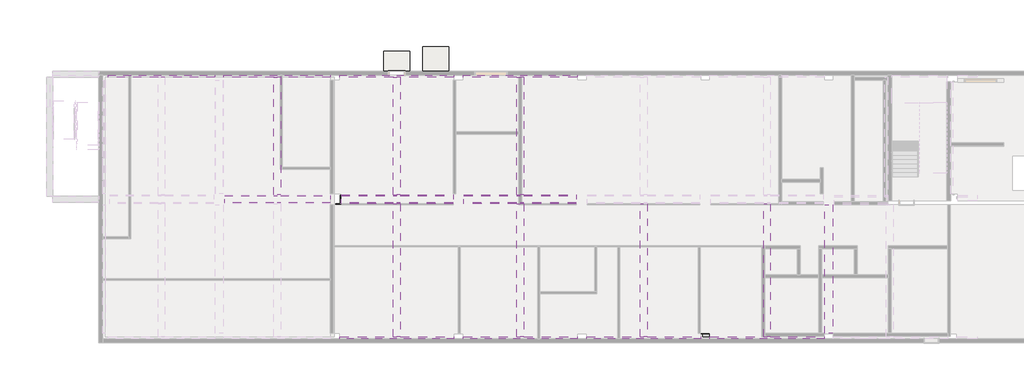
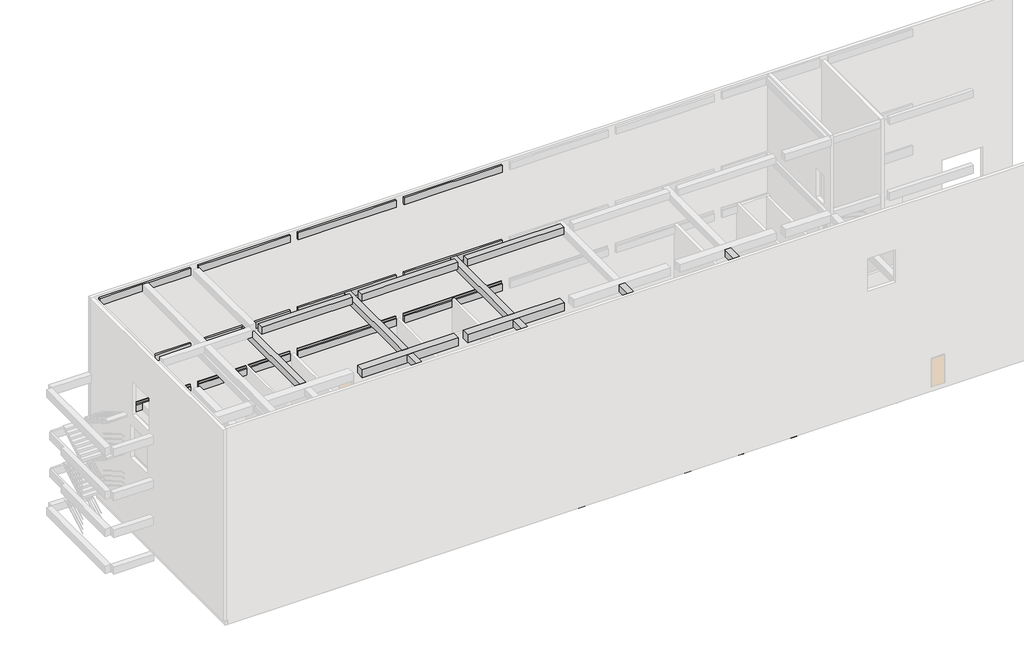
# One storey, part 3 of 5: 54 beams, 2 slabs.
# Revit data of these elements (continued)
# Type "RC Beam_Rectangular : H_SB_AR_S16_UG_B600xH800_1G2" (continued)
#   H_WM Code_1 = "A03AF032-00022 |  | M3 | Concrete Work | Superstructure Work | Structural Concrete | Cement Type-1 | 25MPa ≤ F'c (Cylinder Strength) < 30MPa |  |  |  |  | A03AF032-00022 Concrete Work Superstructure Work Structural Concrete  Cement Type-1 25MPa ≤ F'c (Cylinder Strength) < 30MPa      |  F'c (Cylinder Strength) = 24MPa"
#   H_WM Code_2 = "A03AD037-00002 |  | TON | Concrete Work | Substructure Work | Rebar Work | Deformed Bar (Non-Coat.) | 400MPa<Fy≤470MPa |  |  |  |  | A03AD037-00002 Concrete Work Substructure Work Rebar Work Deformed Bar (Non-Coat.)  400MPa<Fy≤470MPa      | ASTM A615 GRADE 60 (Fy=420MPa)"
#   H_WM Code_3 = "A03AF036-00001 |  | M2 | Concrete Work | Superstructure Work | Form Work (1 time in use) | Flat Form | Dressed Lumber, Plywood or Steel Form(Wood Planks are not Allowed) incl. Chamfer |  |  |  | A03AF036-00001 Concrete Work Superstructure Work Form Work (1 time in use) Flat Form     Dressed Lumber, Plywood or Steel Form(Wood Planks are not Allowed) incl. Chamfer   |"
#   중앙부 하부근 = ""
#   중앙부 상부근 = ""
#   중앙부 보조근 = ""
#   중앙부 늑근 = ""
#   외단부 하부근 = ""
#   외단부 상부근 = ""
#   외단부 보조근 = ""
#   외단부 늑근 = ""
#   부호 = "TG2"
#   내단부 하부근 = ""
#   내단부 상부근 = ""
#   내단부 보조근 = ""
#   내단부 늑근 = ""
#   ALL 하부근 = "3-D20"
#   ALL 상부근 = "4-D20"
#   ALL 보조근 = ""
#   ALL 늑근 = "2-D10 @120"
#   H_Rebar ratio = 0.14
#   Width = 600 mm
#   Height = 800 mm
#   Length [instance default] = 1524 mm
#   b = 600 mm
#   h = 800 mm
#   hec_material3 [instance default] = none
#   hec_material2 [instance default] = none
#   hec_material1 [instance default] = none
#   Structural Material [instance default] = none
#   Assembly Code = ""
# Type "RC Beam_Rectangular : H_SB_AR_S16_UG_B450xH700_1B1"
#   Type Comments = "CV-UG"
#   Type Mark = "1B1"
#   H_Q'ty Cal Type Tag = "SB-Q1"
#   H_WM Code_1 = "A03AF032-00022 |  | M3 | Concrete Work | Superstructure Work | Structural Concrete | Cement Type-1 | 25MPa ≤ F'c (Cylinder Strength) < 30MPa |  |  |  |  | A03AF032-00022 Concrete Work Superstructure Work Structural Concrete  Cement Type-1 25MPa ≤ F'c (Cylinder Strength) < 30MPa      |  F'c (Cylinder Strength) = 24MPa"
#   H_WM Code_2 = "A03AD037-00002 |  | TON | Concrete Work | Substructure Work | Rebar Work | Deformed Bar (Non-Coat.) | 400MPa<Fy≤470MPa |  |  |  |  | A03AD037-00002 Concrete Work Substructure Work Rebar Work Deformed Bar (Non-Coat.)  400MPa<Fy≤470MPa      | ASTM A615 GRADE 60 (Fy=420MPa)"
#   H_WM Code_3 = "A03AF036-00001 |  | M2 | Concrete Work | Superstructure Work | Form Work (1 time in use) | Flat Form | Dressed Lumber, Plywood or Steel Form(Wood Planks are not Allowed) incl. Chamfer |  |  |  | A03AF036-00001 Concrete Work Superstructure Work Form Work (1 time in use) Flat Form     Dressed Lumber, Plywood or Steel Form(Wood Planks are not Allowed) incl. Chamfer   |"
#   중앙부 하부근 = ""
#   중앙부 상부근 = ""
#   중앙부 보조근 = ""
#   중앙부 늑근 = ""
#   외단부 하부근 = ""
#   외단부 상부근 = ""
#   외단부 보조근 = ""
#   외단부 늑근 = ""
#   부호 = "TG2"
#   내단부 하부근 = ""
#   내단부 상부근 = ""
#   내단부 보조근 = ""
#   내단부 늑근 = ""
#   ALL 하부근 = "3-D20"
#   ALL 상부근 = "4-D20"
#   ALL 보조근 = ""
#   ALL 늑근 = "2-D10 @120"
#   H_Rebar ratio = 0.14
#   Width = 450 mm
#   Height = 700 mm
#   Length [instance default] = 1524 mm
#   b = 450 mm
#   h = 700 mm
#   hec_material3 [instance default] = none
#   hec_material2 [instance default] = none
#   hec_material1 [instance default] = none
#   Structural Material [instance default] = none
#   Assembly Code = ""
# Type "RC Beam_Rectangular : H_SB_AR_S16_UG_B500xH700_1G1"
#   Type Comments = "CV-UG"
#   Type Mark = "1G1"
#   H_Q'ty Cal Type Tag = "SB-Q1"
#   H_WM Code_1 = "A03AF032-00022 |  | M3 | Concrete Work | Superstructure Work | Structural Concrete | Cement Type-1 | 25MPa ≤ F'c (Cylinder Strength) < 30MPa |  |  |  |  | A03AF032-00022 Concrete Work Superstructure Work Structural Concrete  Cement Type-1 25MPa ≤ F'c (Cylinder Strength) < 30MPa      |  F'c (Cylinder Strength) = 24MPa"
#   H_WM Code_2 = "A03AD037-00002 |  | TON | Concrete Work | Substructure Work | Rebar Work | Deformed Bar (Non-Coat.) | 400MPa<Fy≤470MPa |  |  |  |  | A03AD037-00002 Concrete Work Substructure Work Rebar Work Deformed Bar (Non-Coat.)  400MPa<Fy≤470MPa      | ASTM A615 GRADE 60 (Fy=420MPa)"
#   H_WM Code_3 = "A03AF036-00001 |  | M2 | Concrete Work | Superstructure Work | Form Work (1 time in use) | Flat Form | Dressed Lumber, Plywood or Steel Form(Wood Planks are not Allowed) incl. Chamfer |  |  |  | A03AF036-00001 Concrete Work Superstructure Work Form Work (1 time in use) Flat Form     Dressed Lumber, Plywood or Steel Form(Wood Planks are not Allowed) incl. Chamfer   |"
#   중앙부 하부근 = ""
#   중앙부 상부근 = ""
#   중앙부 보조근 = ""
#   중앙부 늑근 = ""
#   외단부 하부근 = ""
#   외단부 상부근 = ""
#   외단부 보조근 = ""
#   외단부 늑근 = ""
#   부호 = "TG2"
#   내단부 하부근 = ""
#   내단부 상부근 = ""
#   내단부 보조근 = ""
#   내단부 늑근 = ""
#   ALL 하부근 = "3-D20"
#   ALL 상부근 = "4-D20"
#   ALL 보조근 = ""
#   ALL 늑근 = "2-D10 @120"
#   H_Rebar ratio = 0.14
#   Width = 500 mm
#   Height = 700 mm
#   Length [instance default] = 1524 mm
#   b = 500 mm
#   h = 700 mm
#   hec_material3 [instance default] = none
#   hec_material2 [instance default] = none
#   hec_material1 [instance default] = none
#   Structural Material [instance default] = none
#   Assembly Code = ""
# Type "RC Beam_Rectangular : H_SB_AR_S16_UG_B450xH700_1B1A"
#   Type Comments = "UG"
#   Type Mark = "1B1A"
#   H_Q'ty Cal Type Tag = "SB-Q1"
#   H_WM Code_1 = "A03AF032-00022 |  | M3 | Concrete Work | Superstructure Work | Structural Concrete | Cement Type-1 | 25MPa ≤ F'c (Cylinder Strength) < 30MPa |  |  |  |  | A03AF032-00022 Concrete Work Superstructure Work Structural Concrete  Cement Type-1 25MPa ≤ F'c (Cylinder Strength) < 30MPa      |  F'c (Cylinder Strength) = 24MPa"
#   H_WM Code_2 = "A03AD037-00002 |  | TON | Concrete Work | Substructure Work | Rebar Work | Deformed Bar (Non-Coat.) | 400MPa<Fy≤470MPa |  |  |  |  | A03AD037-00002 Concrete Work Substructure Work Rebar Work Deformed Bar (Non-Coat.)  400MPa<Fy≤470MPa      | ASTM A615 GRADE 60 (Fy=420MPa)"
#   H_WM Code_3 = "A03AF036-00001 |  | M2 | Concrete Work | Superstructure Work | Form Work (1 time in use) | Flat Form | Dressed Lumber, Plywood or Steel Form(Wood Planks are not Allowed) incl. Chamfer |  |  |  | A03AF036-00001 Concrete Work Superstructure Work Form Work (1 time in use) Flat Form     Dressed Lumber, Plywood or Steel Form(Wood Planks are not Allowed) incl. Chamfer   |"
#   중앙부 하부근 = ""
#   중앙부 상부근 = ""
#   중앙부 보조근 = ""
#   중앙부 늑근 = ""
#   외단부 하부근 = ""
#   외단부 상부근 = ""
#   외단부 보조근 = ""
#   외단부 늑근 = ""
#   부호 = "TG2"
#   내단부 하부근 = ""
#   내단부 상부근 = ""
#   내단부 보조근 = ""
#   내단부 늑근 = ""
#   ALL 하부근 = "3-D20"
#   ALL 상부근 = "4-D20"
#   ALL 보조근 = ""
#   ALL 늑근 = "2-D10 @120"
#   Width = 450 mm
#   Height = 700 mm
#   Length [instance default] = 1524 mm
#   b = 450 mm
#   h = 700 mm
#   hec_material3 [instance default] = none
#   hec_material2 [instance default] = none
#   hec_material1 [instance default] = none
#   Structural Material [instance default] = none
#   Assembly Code = ""
# Type "RC Beam_Rectangular : H_SB_AR_S16_AG_B400xH700_3WG1"
#   Type Comments = "CV-AG"
#   Type Mark = "3WG1"
#   H_Q'ty Cal Type Tag = "SB-Q1"
#   H_WM Code_1 = "A03AF032-00022 |  | M3 | Concrete Work | Superstructure Work | Structural Concrete | Cement Type-1 | 25MPa ≤ F'c (Cylinder Strength) < 30MPa |  |  |  |  | A03AF032-00022 Concrete Work Superstructure Work Structural Concrete  Cement Type-1 25MPa ≤ F'c (Cylinder Strength) < 30MPa      |  F'c (Cylinder Strength) = 24MPa"
#   H_WM Code_2 = "A03AD037-00002 |  | TON | Concrete Work | Substructure Work | Rebar Work | Deformed Bar (Non-Coat.) | 400MPa<Fy≤470MPa |  |  |  |  | A03AD037-00002 Concrete Work Substructure Work Rebar Work Deformed Bar (Non-Coat.)  400MPa<Fy≤470MPa      | ASTM A615 GRADE 60 (Fy=420MPa)"
#   H_WM Code_3 = "A03AF036-00001 |  | M2 | Concrete Work | Superstructure Work | Form Work (1 time in use) | Flat Form | Dressed Lumber, Plywood or Steel Form(Wood Planks are not Allowed) incl. Chamfer |  |  |  | A03AF036-00001 Concrete Work Superstructure Work Form Work (1 time in use) Flat Form     Dressed Lumber, Plywood or Steel Form(Wood Planks are not Allowed) incl. Chamfer   |"
#   중앙부 하부근 = ""
#   중앙부 상부근 = ""
#   중앙부 보조근 = ""
#   중앙부 늑근 = ""
#   외단부 하부근 = ""
#   외단부 상부근 = ""
#   외단부 보조근 = ""
#   외단부 늑근 = ""
#   부호 = "TG2"
#   내단부 하부근 = ""
#   내단부 상부근 = ""
#   내단부 보조근 = ""
#   내단부 늑근 = ""
#   ALL 하부근 = "3-D20"
#   ALL 상부근 = "4-D20"
#   ALL 보조근 = ""
#   ALL 늑근 = "2-D10 @120"
#   H_Rebar ratio = 0.14
#   Width = 400 mm
#   Height = 700 mm
#   Length [instance default] = 1524 mm
#   b = 400 mm
#   h = 700 mm
#   hec_material3 [instance default] = none
#   hec_material2 [instance default] = none
#   hec_material1 [instance default] = none
#   Structural Material [instance default] = none
#   Assembly Code = ""
# Type "RC Beam_Rectangular : H_SB_AR_S16_AG_B600xH800_3G2"
#   Type Comments = "AG"
#   Type Mark = "3G2"
#   H_Q'ty Cal Type Tag = "SB-Q1"
#   H_WM Code_1 = "A03AF032-00022 |  | M3 | Concrete Work | Superstructure Work | Structural Concrete | Cement Type-1 | 25MPa ≤ F'c (Cylinder Strength) < 30MPa |  |  |  |  | A03AF032-00022 Concrete Work Superstructure Work Structural Concrete  Cement Type-1 25MPa ≤ F'c (Cylinder Strength) < 30MPa      |  F'c (Cylinder Strength) = 24MPa"
#   H_WM Code_2 = "A03AD037-00002 |  | TON | Concrete Work | Substructure Work | Rebar Work | Deformed Bar (Non-Coat.) | 400MPa<Fy≤470MPa |  |  |  |  | A03AD037-00002 Concrete Work Substructure Work Rebar Work Deformed Bar (Non-Coat.)  400MPa<Fy≤470MPa      | ASTM A615 GRADE 60 (Fy=420MPa)"
#   H_WM Code_3 = "A03AF036-00001 |  | M2 | Concrete Work | Superstructure Work | Form Work (1 time in use) | Flat Form | Dressed Lumber, Plywood or Steel Form(Wood Planks are not Allowed) incl. Chamfer |  |  |  | A03AF036-00001 Concrete Work Superstructure Work Form Work (1 time in use) Flat Form     Dressed Lumber, Plywood or Steel Form(Wood Planks are not Allowed) incl. Chamfer   |"
#   중앙부 하부근 = ""
#   중앙부 상부근 = ""
#   중앙부 보조근 = ""
#   중앙부 늑근 = ""
#   외단부 하부근 = ""
#   외단부 상부근 = ""
#   외단부 보조근 = ""
#   외단부 늑근 = ""
#   부호 = "TG2"
#   내단부 하부근 = ""
#   내단부 상부근 = ""
#   내단부 보조근 = ""
#   내단부 늑근 = ""
#   ALL 하부근 = "3-D20"
#   ALL 상부근 = "4-D20"
#   ALL 보조근 = ""
#   ALL 늑근 = "2-D10 @120"
#   Width = 600 mm
#   Height = 800 mm
#   Length [instance default] = 1524 mm
#   b = 600 mm
#   h = 800 mm
#   hec_material3 [instance default] = none
#   hec_material2 [instance default] = none
#   hec_material1 [instance default] = none
#   Structural Material [instance default] = none
#   Assembly Code = ""
# Type "RC Beam_Rectangular : H_SB_AR_S16_AG_B4500xH700_3G1"
#   Type Comments = "AG"
#   Type Mark = "3G1"
#   H_Q'ty Cal Type Tag = "SB-Q1"
#   H_WM Code_1 = "A03AF032-00022 |  | M3 | Concrete Work | Superstructure Work | Structural Concrete | Cement Type-1 | 25MPa ≤ F'c (Cylinder Strength) < 30MPa |  |  |  |  | A03AF032-00022 Concrete Work Superstructure Work Structural Concrete  Cement Type-1 25MPa ≤ F'c (Cylinder Strength) < 30MPa      |  F'c (Cylinder Strength) = 24MPa"
#   H_WM Code_2 = "A03AD037-00002 |  | TON | Concrete Work | Substructure Work | Rebar Work | Deformed Bar (Non-Coat.) | 400MPa<Fy≤470MPa |  |  |  |  | A03AD037-00002 Concrete Work Substructure Work Rebar Work Deformed Bar (Non-Coat.)  400MPa<Fy≤470MPa      | ASTM A615 GRADE 60 (Fy=420MPa)"
#   H_WM Code_3 = "A03AF036-00001 |  | M2 | Concrete Work | Superstructure Work | Form Work (1 time in use) | Flat Form | Dressed Lumber, Plywood or Steel Form(Wood Planks are not Allowed) incl. Chamfer |  |  |  | A03AF036-00001 Concrete Work Superstructure Work Form Work (1 time in use) Flat Form     Dressed Lumber, Plywood or Steel Form(Wood Planks are not Allowed) incl. Chamfer   |"
#   중앙부 하부근 = ""
#   중앙부 상부근 = ""
#   중앙부 보조근 = ""
#   중앙부 늑근 = ""
#   외단부 하부근 = ""
#   외단부 상부근 = ""
#   외단부 보조근 = ""
#   외단부 늑근 = ""
#   부호 = "TG2"
#   내단부 하부근 = ""
#   내단부 상부근 = ""
#   내단부 보조근 = ""
#   내단부 늑근 = ""
#   ALL 하부근 = "3-D20"
#   ALL 상부근 = "4-D20"
#   ALL 보조근 = ""
#   ALL 늑근 = "2-D10 @120"
#   Width = 500 mm
#   Height = 700 mm
#   Length [instance default] = 1524 mm
#   b = 500 mm
#   h = 700 mm
#   hec_material3 [instance default] = none
#   hec_material2 [instance default] = none
#   hec_material1 [instance default] = none
#   Structural Material [instance default] = none
#   Assembly Code = ""
# Type "RC Beam_Rectangular : H_SB_AR_S16_AG_B450xH700_3B1"
#   Type Comments = "AG"
#   Type Mark = "3B1"
#   H_Q'ty Cal Type Tag = "SB-Q1"
#   H_WM Code_1 = "A03AF032-00022 |  | M3 | Concrete Work | Superstructure Work | Structural Concrete | Cement Type-1 | 25MPa ≤ F'c (Cylinder Strength) < 30MPa |  |  |  |  | A03AF032-00022 Concrete Work Superstructure Work Structural Concrete  Cement Type-1 25MPa ≤ F'c (Cylinder Strength) < 30MPa      |  F'c (Cylinder Strength) = 24MPa"
#   H_WM Code_2 = "A03AD037-00002 |  | TON | Concrete Work | Substructure Work | Rebar Work | Deformed Bar (Non-Coat.) | 400MPa<Fy≤470MPa |  |  |  |  | A03AD037-00002 Concrete Work Substructure Work Rebar Work Deformed Bar (Non-Coat.)  400MPa<Fy≤470MPa      | ASTM A615 GRADE 60 (Fy=420MPa)"
#   H_WM Code_3 = "A03AF036-00001 |  | M2 | Concrete Work | Superstructure Work | Form Work (1 time in use) | Flat Form | Dressed Lumber, Plywood or Steel Form(Wood Planks are not Allowed) incl. Chamfer |  |  |  | A03AF036-00001 Concrete Work Superstructure Work Form Work (1 time in use) Flat Form     Dressed Lumber, Plywood or Steel Form(Wood Planks are not Allowed) incl. Chamfer   |"
#   중앙부 하부근 = ""
#   중앙부 상부근 = ""
#   중앙부 보조근 = ""
#   중앙부 늑근 = ""
#   외단부 하부근 = ""
#   외단부 상부근 = ""
#   외단부 보조근 = ""
#   외단부 늑근 = ""
#   부호 = "TG2"
#   내단부 하부근 = ""
#   내단부 상부근 = ""
#   내단부 보조근 = ""
#   내단부 늑근 = ""
#   ALL 하부근 = "3-D20"
#   ALL 상부근 = "4-D20"
#   ALL 보조근 = ""
#   ALL 늑근 = "2-D10 @120"
#   Width = 450 mm
#   Height = 700 mm
#   Length [instance default] = 1524 mm
#   b = 450 mm
#   h = 700 mm
#   hec_material3 [instance default] = none
#   hec_material2 [instance default] = none
#   hec_material1 [instance default] = none
#   Structural Material [instance default] = none
#   Assembly Code = ""
# Type "RC Beam_Rectangular : H_SB_AR_S16_AG_B450xH700_3B1A"
#   Type Comments = "AG"
#   Type Mark = "3B1A"
#   H_Q'ty Cal Type Tag = "SB-Q1"
#   H_WM Code_1 = "A03AF032-00022 |  | M3 | Concrete Work | Superstructure Work | Structural Concrete | Cement Type-1 | 25MPa ≤ F'c (Cylinder Strength) < 30MPa |  |  |  |  | A03AF032-00022 Concrete Work Superstructure Work Structural Concrete  Cement Type-1 25MPa ≤ F'c (Cylinder Strength) < 30MPa      |  F'c (Cylinder Strength) = 24MPa"
#   H_WM Code_2 = "A03AD037-00002 |  | TON | Concrete Work | Substructure Work | Rebar Work | Deformed Bar (Non-Coat.) | 400MPa<Fy≤470MPa |  |  |  |  | A03AD037-00002 Concrete Work Substructure Work Rebar Work Deformed Bar (Non-Coat.)  400MPa<Fy≤470MPa      | ASTM A615 GRADE 60 (Fy=420MPa)"
#   H_WM Code_3 = "A03AF036-00001 |  | M2 | Concrete Work | Superstructure Work | Form Work (1 time in use) | Flat Form | Dressed Lumber, Plywood or Steel Form(Wood Planks are not Allowed) incl. Chamfer |  |  |  | A03AF036-00001 Concrete Work Superstructure Work Form Work (1 time in use) Flat Form     Dressed Lumber, Plywood or Steel Form(Wood Planks are not Allowed) incl. Chamfer   |"
#   중앙부 하부근 = ""
#   중앙부 상부근 = ""
#   중앙부 보조근 = ""
#   중앙부 늑근 = ""
#   외단부 하부근 = ""
#   외단부 상부근 = ""
#   외단부 보조근 = ""
#   외단부 늑근 = ""
#   부호 = "TG2"
#   내단부 하부근 = ""
#   내단부 상부근 = ""
#   내단부 보조근 = ""
#   내단부 늑근 = ""
#   ALL 하부근 = "3-D20"
#   ALL 상부근 = "4-D20"
#   ALL 보조근 = ""
#   ALL 늑근 = "2-D10 @120"
#   Width = 450 mm
#   Height = 700 mm
#   Length [instance default] = 1524 mm
#   b = 450 mm
#   h = 700 mm
#   hec_material3 [instance default] = none
#   hec_material2 [instance default] = none
#   hec_material1 [instance default] = none
#   Structural Material [instance default] = none
#   Assembly Code = ""
# Type "RC Beam_Rectangular : H_SB_AR_S16_AG_B400xH700_RWG1"
#   Type Comments = "CV-AG"
#   Type Mark = "RWG1"
#   H_Q'ty Cal Type Tag = "SB-Q1"
#   H_WM Code_1 = "A03AF032-00022 |  | M3 | Concrete Work | Superstructure Work | Structural Concrete | Cement Type-1 | 25MPa ≤ F'c (Cylinder Strength) < 30MPa |  |  |  |  | A03AF032-00022 Concrete Work Superstructure Work Structural Concrete  Cement Type-1 25MPa ≤ F'c (Cylinder Strength) < 30MPa      |  F'c (Cylinder Strength) = 24MPa"
#   H_WM Code_2 = "A03AD037-00002 |  | TON | Concrete Work | Substructure Work | Rebar Work | Deformed Bar (Non-Coat.) | 400MPa<Fy≤470MPa |  |  |  |  | A03AD037-00002 Concrete Work Substructure Work Rebar Work Deformed Bar (Non-Coat.)  400MPa<Fy≤470MPa      | ASTM A615 GRADE 60 (Fy=420MPa)"
#   H_WM Code_3 = "A03AF036-00001 |  | M2 | Concrete Work | Superstructure Work | Form Work (1 time in use) | Flat Form | Dressed Lumber, Plywood or Steel Form(Wood Planks are not Allowed) incl. Chamfer |  |  |  | A03AF036-00001 Concrete Work Superstructure Work Form Work (1 time in use) Flat Form     Dressed Lumber, Plywood or Steel Form(Wood Planks are not Allowed) incl. Chamfer   |"
#   중앙부 하부근 = ""
#   중앙부 상부근 = ""
#   중앙부 보조근 = ""
#   중앙부 늑근 = ""
#   외단부 하부근 = ""
#   외단부 상부근 = ""
#   외단부 보조근 = ""
#   외단부 늑근 = ""
#   부호 = "TG2"
#   내단부 하부근 = ""
#   내단부 상부근 = ""
#   내단부 보조근 = ""
#   내단부 늑근 = ""
#   ALL 하부근 = "3-D20"
#   ALL 상부근 = "4-D20"
#   ALL 보조근 = ""
#   ALL 늑근 = "2-D10 @120"
#   H_Rebar ratio = 0.14
#   Width = 400 mm
#   Height = 700 mm
#   Length [instance default] = 1524 mm
#   b = 400 mm
#   h = 700 mm
#   hec_material3 [instance default] = none
#   hec_material2 [instance default] = none
#   hec_material1 [instance default] = none
#   Structural Material [instance default] = none
#   Assembly Code = ""
# Type "RC Beam_Rectangular : H_SB_AR_S16_AG_B450xH700_RG2"
#   Type Comments = "AG"
#   Type Mark = "RG2"
#   H_Q'ty Cal Type Tag = "SB-Q1"
#   H_WM Code_1 = "A03AF032-00022 |  | M3 | Concrete Work | Superstructure Work | Structural Concrete | Cement Type-1 | 25MPa ≤ F'c (Cylinder Strength) < 30MPa |  |  |  |  | A03AF032-00022 Concrete Work Superstructure Work Structural Concrete  Cement Type-1 25MPa ≤ F'c (Cylinder Strength) < 30MPa      |  F'c (Cylinder Strength) = 24MPa"
#   H_WM Code_2 = "A03AD037-00002 |  | TON | Concrete Work | Substructure Work | Rebar Work | Deformed Bar (Non-Coat.) | 400MPa<Fy≤470MPa |  |  |  |  | A03AD037-00002 Concrete Work Substructure Work Rebar Work Deformed Bar (Non-Coat.)  400MPa<Fy≤470MPa      | ASTM A615 GRADE 60 (Fy=420MPa)"
#   H_WM Code_3 = "A03AF036-00001 |  | M2 | Concrete Work | Superstructure Work | Form Work (1 time in use) | Flat Form | Dressed Lumber, Plywood or Steel Form(Wood Planks are not Allowed) incl. Chamfer |  |  |  | A03AF036-00001 Concrete Work Superstructure Work Form Work (1 time in use) Flat Form     Dressed Lumber, Plywood or Steel Form(Wood Planks are not Allowed) incl. Chamfer   |"
#   중앙부 하부근 = ""
#   중앙부 상부근 = ""
#   중앙부 보조근 = ""
#   중앙부 늑근 = ""
#   외단부 하부근 = ""
#   외단부 상부근 = ""
#   외단부 보조근 = ""
#   외단부 늑근 = ""
#   부호 = "TG2"
#   내단부 하부근 = ""
#   내단부 상부근 = ""
#   내단부 보조근 = ""
#   내단부 늑근 = ""
#   ALL 하부근 = "3-D20"
#   ALL 상부근 = "4-D20"
#   ALL 보조근 = ""
#   ALL 늑근 = "2-D10 @120"
#   Width = 450 mm
#   Height = 700 mm
#   Length [instance default] = 1524 mm
#   b = 450 mm
#   h = 700 mm
#   hec_material3 [instance default] = none
#   hec_material2 [instance default] = none
#   hec_material1 [instance default] = none
#   Structural Material [instance default] = none
#   Assembly Code = ""
# Type "H_SF_AR_B08_Ramp_Ramp2"
#   Type Comments = "CV-AG"
#   Type Mark = "Ramp2"
#   H_Q'ty Cal Type Tag = "SB-Q1A"
#   H_WM Code_1 = "A03AF032-00022 |  | M3 | Concrete Work | Superstructure Work | Structural Concrete | Cement Type-1 | 25MPa ≤ F'c (Cylinder Strength) < 30MPa |  |  |  |  | A03AF032-00022 Concrete Work Superstructure Work Structural Concrete  Cement Type-1 25MPa ≤ F'c (Cylinder Strength) < 30MPa      |  F'c (Cylinder Strength) = 24MPa"
#   H_WM Code_2 = "A03AD037-00002 |  | TON | Concrete Work | Substructure Work | Rebar Work | Deformed Bar (Non-Coat.) | 400MPa<Fy≤470MPa |  |  |  |  | A03AD037-00002 Concrete Work Substructure Work Rebar Work Deformed Bar (Non-Coat.)  400MPa<Fy≤470MPa      | ASTM A615 GRADE 60 (Fy=420MPa)"
#   H_WM Code_3 = "A03AD035-00001 |  | M2 | Concrete Work | Substructure Work | Form Work (3 times in use) | Flat Form | Dressed Lumber, Plywood or Steel Form(Wood Planks are not Allowed) incl. Chamfer |  |  |  | A03AD035-00001 Concrete Work Substructure Work Form Work (3 times in use) Flat Form     Dressed Lumber, Plywood or Steel Form(Wood Planks are not Allowed) incl. Chamfer   | Dressed Lumber, Plywood or Steel Form(Wood Planks are not Allowed) incl. Chamfer"
#   H_WM Code_4 = "A03AH056-00001 |  | M2 | Concrete Work | Concrete Protective Coating (U/G) | Bitumen/Bituminous/Asphalt Coating |  |  | A03AH056-00001 Concrete Work Concrete Protective Coating (U/G) Bitumen/Bituminous/Asphalt Coating         | Bitumen/Bituminous/Asphalt Coating"
#   H_WM Code_5 = "A03AD047-00004 |  | M2 | Concrete Work | Substructure Work | Insulation under Ground Floor | Extruded Polystyrene Insulation Board |  | 100mm≤THK | THK=(  )mm |  | A03AD047-00004 Concrete Work Substructure Work Insulation under Ground Floor Extruded Polystyrene Insulation Board       100mm≤THK | Bitumen/Bituminous/Asphalt Coating"
#   H_WM Code_6 = "A01ZZ001-00012 |  | M3 | Earth Work | - | Excavation | Soil, Mech. |  | Manual Excavation Above GWL |  |  |  | A01ZZ001-00012 Earth Work - Excavation Soil, Mech.      Manual Excavation Above GWL  | Above GWL"
#   H_WM Code_7 = "A01ZZ001-00013 |  | M3 | Earth Work | - | Excavation | Soil, Mech. |  | Manual Excavation Below GWL |  |  |  | A01ZZ001-00013 Earth Work - Excavation Soil, Mech.      Manual Excavation Below GWL  | Below GWL"
#   H_WM Code_8 = "A01ZZ003-00001 |  | M3 | Earth Work | - | Backfill | Re-use, Soil |  |  |  | Compaction=(  )% |  | A01ZZ003-00001 Earth Work - Backfill Re-use, Soil        | Compaction=( 95 )%"
#   H_WM Code_9 = "A01ZZ004-00001 |  | M3 | Earth Work | - | Disposal | Soil |  |  |  | Disposal Distance=Appx. (  )km from Site |  | A01ZZ004-00001 Earth Work - Disposal Soil        | Disposal Distance=Appx. (20 )km from Site"
#   H_WM Code_10 = "A03AH056-00001 |  | M2 | Concrete Work | Concrete Protective Coating (U/G) | Bitumen/Bituminous/Asphalt Coating |  |  | A03AH056-00001 Concrete Work Concrete Protective Coating (U/G) Bitumen/Bituminous/Asphalt Coating         | *기초바닥 Protection 은 Lean에 적용"
#   H_Rebar ratio = 0.1
#   Layers, outside or top first: 0 mm no material (function 100); 200 mm "00_Concrete_Reinf. Conc." (function 1); 0 mm no material (function 100); 0 mm no material (function 100)
# Element 1 (IfcBeam, "RC Beam_Rectangular : H_SB_AR_S16_UG_B600xH800_1G2")
#   Comments = ""
#   hec_material3 = none
#   hec_material2 = none
#   hec_material1 = none
#   Structural Material = 00_Concrete_Reinf. Conc.
#   Phase Created = New Construction
#   Materials on its faces: "00_Concrete_Reinf. Conc."
# Elements 2, 3 (IfcBeam, "RC Beam_Rectangular : H_SB_AR_S16_UG_B450xH700_1B1")
#   Comments = ""
#   hec_material3 = none
#   hec_material2 = none
#   hec_material1 = none
#   Structural Material = 00_Concrete_Reinf. Conc.
#   Phase Created = New Construction
#   Materials on its faces: "00_Concrete_Reinf. Conc."
# Elements 4, 5, 6, 7, 8, 9 (IfcBeam, "RC Beam_Rectangular : H_SB_AR_S16_UG_B500xH700_1G1")
#   Comments = ""
#   hec_material3 = none
#   hec_material2 = none
#   hec_material1 = none
#   Structural Material = 00_Concrete_Reinf. Conc.
#   Phase Created = New Construction
#   Materials on its faces: "00_Concrete_Reinf. Conc."
# Elements 10, 11, 12, 13 (IfcBeam, "RC Beam_Rectangular : H_SB_AR_S16_UG_B450xH700_1B1A")
#   Comments = ""
#   hec_material3 = none
#   hec_material2 = none
#   hec_material1 = none
#   Structural Material = none
#   Phase Created = New Construction
# Elements 14, 15, 16, 17, 18, 19, 20, 21, 25, 26, 27, 28, 29, 30, 31, 32 (IfcBeam, "RC Beam_Rectangular : H_SB_AR_S16_AG_B400xH700_3WG1")
#   Comments = ""
#   hec_material3 = none
#   hec_material2 = none
#   hec_material1 = none
#   Structural Material = 00_Concrete_Reinf. Conc.
#   Phase Created = New Construction
#   Materials on its faces: "00_Concrete_Reinf. Conc."
# Elements 22, 23, 33, 34 (IfcBeam, "RC Beam_Rectangular : H_SB_AR_S16_AG_B600xH800_3G2")
#   Comments = ""
#   hec_material3 = none
#   hec_material2 = none
#   hec_material1 = none
#   Structural Material = none
#   Phase Created = New Construction
# Element 24 (IfcBeam, "RC Beam_Rectangular : H_SB_AR_S16_AG_B4500xH700_3G1")
#   Comments = ""
#   hec_material3 = none
#   hec_material2 = none
#   hec_material1 = none
#   Structural Material = none
#   Phase Created = New Construction
# Elements 35, 36, 37 (IfcBeam, "RC Beam_Rectangular : H_SB_AR_S16_AG_B450xH700_3B1")
#   Comments = ""
#   hec_material3 = none
#   hec_material2 = none
#   hec_material1 = none
#   Structural Material = none
#   Phase Created = New Construction
# Elements 38, 39, 40, 41 (IfcBeam, "RC Beam_Rectangular : H_SB_AR_S16_AG_B450xH700_3B1A")
#   Comments = ""
#   hec_material3 = none
#   hec_material2 = none
#   hec_material1 = none
#   Structural Material = none
#   Phase Created = New Construction
# Elements 42, 43, 44, 45, 46, 47, 48, 49 (IfcBeam, "RC Beam_Rectangular : H_SB_AR_S16_AG_B400xH700_RWG1")
#   Comments = ""
#   hec_material3 = none
#   hec_material2 = none
#   hec_material1 = none
#   Structural Material = 00_Concrete_Reinf. Conc.
#   Phase Created = New Construction
#   Materials on its faces: "00_Concrete_Reinf. Conc."
# Elements 50, 51, 52 (IfcBeam, "RC Beam_Rectangular : H_SB_AR_S16_AG_B450xH700_RG2")
#   Comments = ""
#   hec_material3 = none
#   hec_material2 = none
#   hec_material1 = none
#   Structural Material = none
#   Phase Created = New Construction
# Element 53 (IfcBeam, "RC Beam_Rectangular : H_SB_AR_S16_UG_B600xH800_1G2")
#   IfcGUID = "0DKOmQSjf1KgvfYSs63FG0"
#   Comments = ""
#   Phase Created = New Construction
#   Materials on its faces: "00_Concrete_Reinf. Conc."
# Element 54 (IfcBeam, "RC Beam_Rectangular : H_SB_AR_S16_UG_B600xH800_1G2")
#   IfcGUID = "0DKOmQSjf1KgvfYSs63FHI"
#   Comments = ""
#   Phase Created = New Construction
#   Materials on its faces: "00_Concrete_Reinf. Conc."
# Elements 55, 56 (IfcSlab, "H_SF_AR_B08_Ramp_Ramp2")
#   Comments = ""
#   built-in parameter 1001955 = 3.14159 (stored number, unit not read)
#   Height Offset From Level = 0 mm
#   built-in parameter 1001954 = 1
#   Phase Created = New Construction
# Materials
#   "00_Concrete_Reinf. Conc.": class "Concrete", colour RGB 176 176 176, transparency 0, Description = "Reinf. Conc.", Cost = 0, Image = Concrete.Cast-In-Place.Flat.Polished.Grey.jpg
# Room at (48881.519, 2598.242) mm, phase "New Construction", upper level "TOC", upper offset 2700 mm, lower offset 0 mm
#   Comments = ""
#   Number = "121"
#   Name = "TOILET (M)"
#   H_Floor Finish Style Name = "Non-Slip Unglazed Ceramic Tile"
#   H_Floor Base Material = "Concrete Slab / Screed / Liquid Waterproofing"
#   H_Wall-Base Material-1 = "Masonry Wall"
#   H_Wall-Base Material-2 = ""
#   H_Wall-Base Material-3 = ""
#   H_Floor-Base Material-1 = "Concrete Slab"
#   H_Floor-Base Material-2 = ""
#   H_Floor-Base Material-3 = "Screed"
#   H_Floor-Base Material-4 = "Concrete Slab"
#   H_Floor-Base Material-5 = ""
#   H_Floor Finish-1 = "Screed"
#   H_Floor Finish-2 = "Liquid Waterproofing"
#   H_Floor Finish Remark = "Ceramic Tile"
#   H_Wall Finish Style Name = "Glazed Ceramic Tile"
#   H_Wall Base Material = "Masonry Wall"
#   H_Wall-Base Material-4 = "Liquid Waterproofing"
#   H_Wall-Base Material-5 = "Glazed Ceramic Tile"
#   H_Wall Finish-1 = "Glazed Ceramic Tile"
#   H_Wall Finish-2 = ""
#   H_Ceiling Finish Style Name = "Suspended Moisture Resistant Tiled Ceiling (M-Bar)"
#   H_Ceiling Base Material = "Concrete Slab / Fair Faced Concrete"
#   H_Ceiling-Base Material-1 = "(Concrete Slab)"
#   H_Ceiling-Base Material-2 = "(Fair Faced Concrete)"
#   H_Ceiling-Base Material-3 = ""
#   H_Ceiling-Base Material-4 = ""
#   H_Ceiling-Base Material-5 = "Moisture Resistant Tiled Ceiling System (M-Bar)"
#   H_Ceiling Finish-1 = "Moisture Resistant Tiled Ceiling System (M-Bar)"
#   H_Ceiling Finish-2 = ""
#   H_Room W = 3800 mm
#   H_Room L = 5600 mm
#   H_Room H or CH = 2700 mm
#   Floor Finish Style No = F31B
#   Wall Finish Style No = W34B
#   Ceiling Finish Style No = C96A
# Room at (40583.851, 3309.471) mm, phase "New Construction", upper level "TOC", upper offset 3000 mm, lower offset 0 mm
#   Comments = ""
#   Number = "117"
#   Name = "PARTNER'S ROOM"
#   H_Floor Finish Style Name = "Vinyl Tile"
#   H_Floor Base Material = "Concrete Slab / Steel Trowel Finish"
#   H_Wall-Base Material-1 = "Concrete Wall"
#   H_Skirt Finish Style Name = "Coved Vinyl Tile"
#   H_Wall-Base Material-2 = "(Fair Faced Concrete)"
#   H_Wall-Base Material-3 = ""
#   H_Floor-Base Material-1 = "Concrete Slab"
#   H_Floor-Base Material-2 = "Steel Trowel Finish"
#   H_Floor-Base Material-3 = ""
#   H_Floor-Base Material-4 = "Concrete Slab"
#   H_Floor-Base Material-5 = "Steel Trowel Finish"
#   H_Floor Finish-1 = ""
#   H_Floor Finish-2 = ""
#   H_Floor Finish Remark = "Vinyl Tile"
#   H_Skirt Base Material = "Same as Wall"
#   H_Skirt-Base Material-1 = ""
#   H_Skirt-Base Material-2 = ""
#   H_Skirt-Base Material-3 = ""
#   H_Skirt-Base Material-4 = ""
#   H_Skirt-Base Material-5 = ""
#   H_Skirt Finish-1 = "Vinyl Tile"
#   H_Skirt Finish-2 = ""
#   H_Wall Finish Style Name = "Water Emulsion Paint"
#   H_Wall Base Material = "Masonry Wall / Cement Plaster"
#   H_Wall-Base Material-4 = ""
#   H_Wall-Base Material-5 = ""
#   H_Wall Finish-1 = "Water Emulsion Paint"
#   H_Wall Finish-2 = ""
#   H_Ceiling Finish Style Name = "Suspended Acoustic Tiled Ceiling (M-Bar)"
#   H_Ceiling Base Material = "Concrete Slab / Fair Faced Concrete"
#   H_Ceiling-Base Material-1 = "(Concrete Slab)"
#   H_Ceiling-Base Material-2 = "(Fair Faced Concrete)"
#   H_Ceiling-Base Material-3 = ""
#   H_Ceiling-Base Material-4 = ""
#   H_Ceiling-Base Material-5 = "Acoustic Tiled Ceiling System (M-Bar)"
#   H_Ceiling Finish-1 = "Acoustic Tiled Ceiling System (M-Bar)"
#   H_Ceiling Finish-2 = ""
#   H_Room W = 3700 mm
#   H_Room L = 3700 mm
#   H_Room H or CH = 3000 mm
#   Floor Finish Style No = F34A
#   Skirt Finish Style No = B35
#   Wall Finish Style No = W02A
#   Ceiling Finish Style No = C95A
# Room at (25580.312, 3648.151) mm, phase "New Construction", upper level "TOC", upper offset 3000 mm, lower offset 0 mm
#   Comments = ""
#   Number = "115"
#   Name = "REST ROOM"
#   H_Floor Finish Style Name = "Vinyl Tile"
#   H_Floor Base Material = "Concrete Slab / Screed"
#   H_Wall-Base Material-1 = "Concrete Wall"
#   H_Skirt Finish Style Name = "Coved Vinyl Tile"
#   H_Wall-Base Material-2 = "(Fair Faced Concrete)"
#   H_Wall-Base Material-3 = ""
#   H_Floor-Base Material-1 = "Concrete Slab"
#   H_Floor-Base Material-2 = "Steel Trowel Finish"
#   H_Floor-Base Material-3 = ""
#   H_Floor-Base Material-4 = "Concrete Slab"
#   H_Floor-Base Material-5 = ""
#   H_Floor Finish-1 = "Screed"
#   H_Floor Finish-2 = ""
#   H_Floor Finish Remark = "Vinyl Tile"
#   H_Skirt Base Material = "Same as Wall"
#   H_Skirt-Base Material-1 = ""
#   H_Skirt-Base Material-2 = ""
#   H_Skirt-Base Material-3 = ""
#   H_Skirt-Base Material-4 = ""
#   H_Skirt-Base Material-5 = ""
#   H_Skirt Finish-1 = "Vinyl Tile"
#   H_Skirt Finish-2 = ""
#   H_Wall Finish Style Name = "Water Emulsion Paint"
#   H_Wall Base Material = "Masonry Wall / Cement Plaster"
#   H_Wall-Base Material-4 = ""
#   H_Wall-Base Material-5 = ""
#   H_Wall Finish-1 = "Water Emulsion Paint"
#   H_Wall Finish-2 = ""
#   H_Ceiling Finish Style Name = "Suspended Gypsum Plaster Board Ceiling (M-Bar)"
#   H_Ceiling Base Material = "Concrete Slab / Fair Faced Concrete"
#   H_Ceiling-Base Material-1 = "(Concrete Slab)"
#   H_Ceiling-Base Material-2 = "(Fair Faced Concrete)"
#   H_Ceiling-Base Material-3 = ""
#   H_Ceiling-Base Material-4 = ""
#   H_Ceiling-Base Material-5 = "Gypsum Plaster Board Ceiling System"
#   H_Ceiling Finish-1 = "Gypsum Plaster Board Ceiling System"
#   H_Ceiling Finish-2 = ""
#   H_Room W = 3700 mm
#   H_Room L = 3000 mm
#   H_Room H or CH = 3000 mm
#   Floor Finish Style No = F34B
#   Skirt Finish Style No = B35
#   Wall Finish Style No = W02A
#   Ceiling Finish Style No = C92
# Room at (6490.87, 11650.959) mm, phase "New Construction", upper level "TOC", upper offset 3000 mm, lower offset -700 mm
#   Comments = ""
#   Number = "101"
#   Name = "CENTRAL CONTROL ROOM"
#   H_Floor Finish Style Name = "Anti-Dust Epoxy Paint / Anti-Static Vinyl Tile on Raised Floor"
#   H_Floor Base Material = "Concrete Slab / Steel Trowel Finish"
#   H_Wall-Base Material-1 = "Concrete Wall"
#   H_Skirt Finish Style Name = "Coved Vinyl Tile"
#   H_Wall-Base Material-2 = "(Fair Faced Concrete)"
#   H_Wall-Base Material-3 = ""
#   H_Floor-Base Material-1 = "Concrete Slab"
#   H_Floor-Base Material-2 = "Steel Trowel Finish"
#   H_Floor-Base Material-3 = ""
#   H_Floor-Base Material-4 = "Concrete Slab"
#   H_Floor-Base Material-5 = "Steel Trowel Finish"
#   H_Floor Finish-1 = ""
#   H_Floor Finish-2 = "Anti-Dust Paint"
#   H_Floor Finish Remark = "Raised Floor_Anti-Static Vinyl Tile"
#   H_Skirt Base Material = "Same as Wall"
#   H_Skirt-Base Material-1 = ""
#   H_Skirt-Base Material-2 = ""
#   H_Skirt-Base Material-3 = ""
#   H_Skirt-Base Material-4 = ""
#   H_Skirt-Base Material-5 = ""
#   H_Skirt Finish-1 = "Vinyl Tile"
#   H_Skirt Finish-2 = ""
#   H_Wall Finish Style Name = "Water Emulsion Paint"
#   H_Wall Base Material = "Masonry Wall / Cement Plaster"
#   H_Wall-Base Material-4 = ""
#   H_Wall-Base Material-5 = ""
#   H_Wall Finish-1 = "Water Emulsion Paint"
#   H_Wall Finish-2 = ""
#   H_Ceiling Finish Style Name = "Suspended Acoustic Tiled Ceiling (M-Bar)"
#   H_Ceiling Base Material = "Concrete Slab / Fair Faced Concrete"
#   H_Ceiling-Base Material-1 = "(Concrete Slab)"
#   H_Ceiling-Base Material-2 = "(Fair Faced Concrete)"
#   H_Ceiling-Base Material-3 = ""
#   H_Ceiling-Base Material-4 = ""
#   H_Ceiling-Base Material-5 = "Acoustic Tiled Ceiling System (M-Bar)"
#   H_Ceiling Finish-1 = "Acoustic Tiled Ceiling System (M-Bar)"
#   H_Ceiling Finish-2 = ""
#   H_Floor Finish Style No = "Concrete Tile"
#   H_Room W = 14900 mm
#   H_Room L = 13300 mm
#   H_Room H or CH = 3000 mm
#   Floor Finish Style No = F91
#   Skirt Finish Style No = B35
#   Wall Finish Style No = W02A
#   Ceiling Finish Style No = C95A
# Room at (904.971, 12877.131) mm, phase "New Construction", upper level "TOC", upper offset 5800 mm, lower offset -700 mm
#   Comments = ""
#   Number = "127"
#   Name = "NONE"
#   H_Floor Finish Style Name = "Anti-Dust Epoxy Paint / Anti-Static Vinyl Tile on Raised Floor"
#   H_Floor Base Material = "Concrete Slab / Steel Trowel Finish"
#   H_Wall-Base Material-1 = "Concrete Wall"
#   H_Skirt Finish Style Name = "Coved Vinyl Tile"
#   H_Wall-Base Material-2 = "(Fair Faced Concrete)"
#   H_Wall-Base Material-3 = ""
#   H_Floor-Base Material-1 = "Concrete Slab"
#   H_Floor-Base Material-2 = "Steel Trowel Finish"
#   H_Floor-Base Material-3 = ""
#   H_Floor-Base Material-4 = "Concrete Slab"
#   H_Floor-Base Material-5 = "Steel Trowel Finish"
#   H_Floor Finish-1 = ""
#   H_Floor Finish-2 = "Anti-Dust Paint"
#   H_Floor Finish Remark = "Raised Floor_Anti-Static Vinyl Tile"
#   H_Skirt Base Material = "Same as Wall"
#   H_Skirt-Base Material-1 = ""
#   H_Skirt-Base Material-2 = ""
#   H_Skirt-Base Material-3 = ""
#   H_Skirt-Base Material-4 = ""
#   H_Skirt-Base Material-5 = ""
#   H_Skirt Finish-1 = "Vinyl Tile"
#   H_Skirt Finish-2 = ""
#   H_Wall Finish Style Name = "Water Emulsion Paint"
#   H_Wall Base Material = "Masonry Wall / Cement Plaster"
#   H_Wall-Base Material-4 = ""
#   H_Wall-Base Material-5 = ""
#   H_Wall Finish-1 = "Water Emulsion Paint"
#   H_Wall Finish-2 = ""
#   H_Ceiling Finish Style Name = "Suspended Acoustic Tiled Ceiling (M-Bar)"
#   H_Ceiling Base Material = "Concrete Slab / Fair Faced Concrete"
#   H_Ceiling-Base Material-1 = "(Concrete Slab)"
#   H_Ceiling-Base Material-2 = "(Fair Faced Concrete)"
#   H_Ceiling-Base Material-3 = ""
#   H_Ceiling-Base Material-4 = ""
#   H_Ceiling-Base Material-5 = "Acoustic Tiled Ceiling System (M-Bar)"
#   H_Ceiling Finish-1 = "Acoustic Tiled Ceiling System (M-Bar)"
#   H_Ceiling Finish-2 = ""
#   H_Room W = 700 mm
#   H_Room L = 700 mm
#   H_Room H or CH = 3000 mm
#   Floor Finish Style No = F91
#   Skirt Finish Style No = B35
#   Wall Finish Style No = W02A
#   Ceiling Finish Style No = C95A
# Room at (13098.579, 14171.425) mm, phase "New Construction", upper level "TOC", upper offset 3000 mm, lower offset -700 mm
#   Comments = ""
#   Number = "102"
#   Name = "MEETING ROOM"
#   H_Floor Finish Style Name = "Anti-Dust Epoxy Paint / Anti-Static Vinyl Tile on Raised Floor"
#   H_Floor Base Material = "Concrete Slab / Steel Trowel Finish"
#   H_Wall-Base Material-1 = "Concrete Wall"
#   H_Skirt Finish Style Name = "Coved Vinyl Tile"
#   H_Wall-Base Material-2 = "(Fair Faced Concrete)"
#   H_Wall-Base Material-3 = ""
#   H_Floor-Base Material-1 = "Concrete Slab"
#   H_Floor-Base Material-2 = "Steel Trowel Finish"
#   H_Floor-Base Material-3 = ""
#   H_Floor-Base Material-4 = "Concrete Slab"
#   H_Floor-Base Material-5 = "Steel Trowel Finish"
#   H_Floor Finish-1 = ""
#   H_Floor Finish-2 = "Anti-Dust Paint"
#   H_Floor Finish Remark = "Raised Floor_Anti-Static Vinyl Tile"
#   H_Skirt Base Material = "Same as Wall"
#   H_Skirt-Base Material-1 = ""
#   H_Skirt-Base Material-2 = ""
#   H_Skirt-Base Material-3 = ""
#   H_Skirt-Base Material-4 = ""
#   H_Skirt-Base Material-5 = ""
#   H_Skirt Finish-1 = "Vinyl Tile"
#   H_Skirt Finish-2 = ""
#   H_Wall Finish Style Name = "Water Emulsion Paint"
#   H_Wall Base Material = "Masonry Wall / Cement Plaster"
#   H_Wall-Base Material-4 = ""
#   H_Wall-Base Material-5 = ""
#   H_Wall Finish-1 = "Water Emulsion Paint"
#   H_Wall Finish-2 = ""
#   H_Ceiling Finish Style Name = "Suspended Acoustic Tiled Ceiling (M-Bar)"
#   H_Ceiling Base Material = "Concrete Slab / Fair Faced Concrete"
#   H_Ceiling-Base Material-1 = "(Concrete Slab)"
#   H_Ceiling-Base Material-2 = "(Fair Faced Concrete)"
#   H_Ceiling-Base Material-3 = ""
#   H_Ceiling-Base Material-4 = ""
#   H_Ceiling-Base Material-5 = "Acoustic Tiled Ceiling System (M-Bar)"
#   H_Ceiling Finish-1 = "Acoustic Tiled Ceiling System (M-Bar)"
#   H_Ceiling Finish-2 = ""
#   H_Floor Finish Style No = "Acrylic Emulsion Paint"
#   H_Room W = 1800 mm
#   H_Room L = 10600 mm
#   H_Room H or CH = 3000 mm
#   Floor Finish Style No = F91
#   Skirt Finish Style No = B35
#   Wall Finish Style No = W02A
#   Ceiling Finish Style No = C95A
# Room at (6967.715, 2863.387) mm, phase "New Construction", upper level "TOC", upper offset 3000 mm, lower offset -700 mm
#   Comments = ""
#   Number = "103"
#   Name = "ENGINEERING ROOM"
#   H_Floor Finish Style Name = "Anti-Dust Epoxy Paint / Anti-Static Vinyl Tile on Raised Floor"
#   H_Floor Base Material = "Concrete Slab / Steel Trowel Finish"
#   H_Wall-Base Material-1 = "Concrete Wall"
#   H_Skirt Finish Style Name = "Coved Vinyl Tile"
#   H_Wall-Base Material-2 = "(Fair Faced Concrete)"
#   H_Wall-Base Material-3 = ""
#   H_Floor-Base Material-1 = "Concrete Slab"
#   H_Floor-Base Material-2 = "Steel Trowel Finish"
#   H_Floor-Base Material-3 = ""
#   H_Floor-Base Material-4 = "Concrete Slab"
#   H_Floor-Base Material-5 = "Steel Trowel Finish"
#   H_Floor Finish-1 = ""
#   H_Floor Finish-2 = "Anti-Dust Paint"
#   H_Floor Finish Remark = "Raised Floor_Anti-Static Vinyl Tile"
#   H_Skirt Base Material = "Same as Wall"
#   H_Skirt-Base Material-1 = ""
#   H_Skirt-Base Material-2 = ""
#   H_Skirt-Base Material-3 = ""
#   H_Skirt-Base Material-4 = ""
#   H_Skirt-Base Material-5 = ""
#   H_Skirt Finish-1 = "Vinyl Tile"
#   H_Skirt Finish-2 = ""
#   H_Wall Finish Style Name = "Water Emulsion Paint"
#   H_Wall Base Material = "Masonry Wall / Cement Plaster"
#   H_Wall-Base Material-4 = ""
#   H_Wall-Base Material-5 = ""
#   H_Wall Finish-1 = "Water Emulsion Paint"
#   H_Wall Finish-2 = ""
#   H_Ceiling Finish Style Name = "Suspended Acoustic Tiled Ceiling (M-Bar)"
#   H_Ceiling Base Material = "Concrete Slab / Fair Faced Concrete"
#   H_Ceiling-Base Material-1 = "(Concrete Slab)"
#   H_Ceiling-Base Material-2 = "(Fair Faced Concrete)"
#   H_Ceiling-Base Material-3 = ""
#   H_Ceiling-Base Material-4 = ""
#   H_Ceiling-Base Material-5 = "Acoustic Tiled Ceiling System (M-Bar)"
#   H_Ceiling Finish-1 = "Acoustic Tiled Ceiling System (M-Bar)"
#   H_Ceiling Finish-2 = ""
#   H_Room W = 3200 mm
#   H_Room L = 6100 mm
#   H_Room H or CH = 3000 mm
#   Floor Finish Style No = F91
#   Skirt Finish Style No = B35
#   Wall Finish Style No = W02A
#   Ceiling Finish Style No = C95A
# Room at (18684.477, 14171.425) mm, phase "New Construction", upper level "TOC", upper offset 3000 mm, lower offset 0 mm
#   Comments = ""
#   Number = "104"
#   Name = "CANTEEN"
#   H_Floor Finish Style Name = "Vinyl Tile"
#   H_Floor Base Material = "Concrete Slab / Screed"
#   H_Wall-Base Material-1 = "Concrete Wall"
#   H_Skirt Finish Style Name = "Coved Vinyl Tile"
#   H_Wall-Base Material-2 = "(Fair Faced Concrete)"
#   H_Wall-Base Material-3 = ""
#   H_Floor-Base Material-1 = "Concrete Slab"
#   H_Floor-Base Material-2 = ""
#   H_Floor-Base Material-3 = "Screed"
#   H_Floor-Base Material-4 = "Concrete Slab"
#   H_Floor-Base Material-5 = ""
#   H_Floor Finish-1 = "Screed"
#   H_Floor Finish-2 = ""
#   H_Floor Finish Remark = "Vinyl Tile"
#   H_Skirt Base Material = "Same as Wall"
#   H_Skirt-Base Material-1 = ""
#   H_Skirt-Base Material-2 = ""
#   H_Skirt-Base Material-3 = ""
#   H_Skirt-Base Material-4 = ""
#   H_Skirt-Base Material-5 = ""
#   H_Skirt Finish-1 = "Vinyl Tile"
#   H_Skirt Finish-2 = ""
#   H_Wall Finish Style Name = "Water Emulsion Paint"
#   H_Wall Base Material = "Masonry Wall / Cement Plaster"
#   H_Wall-Base Material-4 = ""
#   H_Wall-Base Material-5 = ""
#   H_Wall Finish-1 = "Water Emulsion Paint"
#   H_Wall Finish-2 = ""
#   H_Ceiling Finish Style Name = "Suspended Gypsum Plaster Board Ceiling (M-Bar)"
#   H_Ceiling Base Material = "Concrete Slab / Fair Faced Concrete"
#   H_Ceiling-Base Material-1 = "(Concrete Slab)"
#   H_Ceiling-Base Material-2 = "(Fair Faced Concrete)"
#   H_Ceiling-Base Material-3 = ""
#   H_Ceiling-Base Material-4 = ""
#   H_Ceiling-Base Material-5 = "Gypsum Plaster Board Ceiling System"
#   H_Ceiling Finish-1 = "Gypsum Plaster Board Ceiling System"
#   H_Ceiling Finish-2 = ""
#   H_Room W = 14900 mm
#   H_Room L = 3900 mm
#   H_Room H or CH = 3000 mm
#   Floor Finish Style No = F34B
#   Skirt Finish Style No = B35
#   Wall Finish Style No = W02A
#   Ceiling Finish Style No = C92
# Room at (24679.1, 15942.564) mm, phase "New Construction", upper level "TOC", upper offset 3000 mm, lower offset 0 mm
#   Comments = ""
#   Number = "105"
#   Name = "AIR LOCK"
#   H_Floor Finish Style Name = "Porcelain Tile"
#   H_Floor Base Material = "Concrete Slab / Steel Trowel Finish"
#   H_Wall-Base Material-1 = "Concrete Wall"
#   H_Skirt Finish Style Name = "Coved Vinyl Tile"
#   H_Wall-Base Material-2 = "(Fair Faced Concrete)"
#   H_Wall-Base Material-3 = ""
#   H_Floor-Base Material-1 = "Concrete Slab"
#   H_Floor-Base Material-2 = "Steel Trowel Finish"
#   H_Floor-Base Material-3 = ""
#   H_Floor-Base Material-4 = "Concrete Slab"
#   H_Floor-Base Material-5 = "Steel Trowel Finish"
#   H_Floor Finish-1 = ""
#   H_Floor Finish-2 = ""
#   H_Floor Finish Remark = "Porcelain Tile"
#   H_Skirt Base Material = "Same as Wall"
#   H_Skirt-Base Material-1 = ""
#   H_Skirt-Base Material-2 = ""
#   H_Skirt-Base Material-3 = ""
#   H_Skirt-Base Material-4 = ""
#   H_Skirt-Base Material-5 = ""
#   H_Skirt Finish-1 = "Vinyl Tile"
#   H_Skirt Finish-2 = ""
#   H_Wall Finish Style Name = "Water Emulsion Paint"
#   H_Wall Base Material = "Masonry Wall / Cement Plaster"
#   H_Wall-Base Material-4 = ""
#   H_Wall-Base Material-5 = ""
#   H_Wall Finish-1 = "Water Emulsion Paint"
#   H_Wall Finish-2 = ""
#   H_Ceiling Finish Style Name = "Suspended Gypsum Plaster Board Ceiling (M-Bar)"
#   H_Ceiling Base Material = "Concrete Slab / Fair Faced Concrete"
#   H_Ceiling-Base Material-1 = "(Concrete Slab)"
#   H_Ceiling-Base Material-2 = "(Fair Faced Concrete)"
#   H_Ceiling-Base Material-3 = ""
#   H_Ceiling-Base Material-4 = ""
#   H_Ceiling-Base Material-5 = "Gypsum Plaster Board Ceiling System"
#   H_Ceiling Finish-1 = "Gypsum Plaster Board Ceiling System"
#   H_Ceiling Finish-2 = ""
#   H_Room W = 7900 mm
#   H_Room L = 8400 mm
#   H_Room H or CH = 3000 mm
#   Floor Finish Style No = F41
#   Skirt Finish Style No = B35
#   Wall Finish Style No = W02A
#   Ceiling Finish Style No = C92
# Room at (24679.1, 11446.597) mm, phase "New Construction", upper level "TOC", upper offset 3000 mm, lower offset 0 mm
#   Comments = ""
#   Number = "106"
#   Name = "LOBBY"
#   H_Floor Finish Style Name = "Vinyl Tile"
#   H_Floor Base Material = "Concrete Slab / Steel Trowel Finish"
#   H_Wall-Base Material-1 = "Concrete Wall"
#   H_Skirt Finish Style Name = "Coved Vinyl Tile"
#   H_Wall-Base Material-2 = "(Fair Faced Concrete)"
#   H_Wall-Base Material-3 = ""
#   H_Floor-Base Material-1 = "Concrete Slab"
#   H_Floor-Base Material-2 = "Steel Trowel Finish"
#   H_Floor-Base Material-3 = ""
#   H_Floor-Base Material-4 = "Concrete Slab"
#   H_Floor-Base Material-5 = "Steel Trowel Finish"
#   H_Floor Finish-1 = ""
#   H_Floor Finish-2 = ""
#   H_Floor Finish Remark = "Vinyl Tile"
#   H_Skirt Base Material = "Same as Wall"
#   H_Skirt-Base Material-1 = ""
#   H_Skirt-Base Material-2 = ""
#   H_Skirt-Base Material-3 = ""
#   H_Skirt-Base Material-4 = ""
#   H_Skirt-Base Material-5 = ""
#   H_Skirt Finish-1 = "Vinyl Tile"
#   H_Skirt Finish-2 = ""
#   H_Wall Finish Style Name = "Water Emulsion Paint"
#   H_Wall Base Material = "Masonry Wall / Cement Plaster"
#   H_Wall-Base Material-4 = ""
#   H_Wall-Base Material-5 = ""
#   H_Wall Finish-1 = "Water Emulsion Paint"
#   H_Wall Finish-2 = ""
#   H_Ceiling Finish Style Name = "Suspended Gypsum Plaster Board Ceiling (M-Bar)"
#   H_Ceiling Base Material = "Concrete Slab / Fair Faced Concrete"
#   H_Ceiling-Base Material-1 = "(Concrete Slab)"
#   H_Ceiling-Base Material-2 = "(Fair Faced Concrete)"
#   H_Ceiling-Base Material-3 = ""
#   H_Ceiling-Base Material-4 = ""
#   H_Ceiling-Base Material-5 = "Gypsum Plaster Board Ceiling System"
#   H_Ceiling Finish-1 = "Gypsum Plaster Board Ceiling System"
#   H_Ceiling Finish-2 = ""
#   H_Room W = 4200 mm
#   H_Room L = 3800 mm
#   H_Room H or CH = 3000 mm
#   Floor Finish Style No = F34A
#   Skirt Finish Style No = B35
#   Wall Finish Style No = W02A
#   Ceiling Finish Style No = C92
# Room at (34859.74, 12931.628) mm, phase "New Construction", upper level "TOC", upper offset 3000 mm, lower offset 0 mm
#   Comments = ""
#   Number = "107"
#   Name = "OFFICE ROOM"
#   H_Floor Finish Style Name = "Vinyl Tile"
#   H_Floor Base Material = "Concrete Slab / Steel Trowel Finish"
#   H_Wall-Base Material-1 = "Concrete Wall"
#   H_Skirt Finish Style Name = "Coved Vinyl Tile"
#   H_Wall-Base Material-2 = "(Fair Faced Concrete)"
#   H_Wall-Base Material-3 = ""
#   H_Floor-Base Material-1 = "Concrete Slab"
#   H_Floor-Base Material-2 = "Steel Trowel Finish"
#   H_Floor-Base Material-3 = ""
#   H_Floor-Base Material-4 = "Concrete Slab"
#   H_Floor-Base Material-5 = "Steel Trowel Finish"
#   H_Floor Finish-1 = ""
#   H_Floor Finish-2 = ""
#   H_Floor Finish Remark = "Vinyl Tile"
#   H_Skirt Base Material = "Same as Wall"
#   H_Skirt-Base Material-1 = ""
#   H_Skirt-Base Material-2 = ""
#   H_Skirt-Base Material-3 = ""
#   H_Skirt-Base Material-4 = ""
#   H_Skirt-Base Material-5 = ""
#   H_Skirt Finish-1 = "Vinyl Tile"
#   H_Skirt Finish-2 = ""
#   H_Wall Finish Style Name = "Water Emulsion Paint"
#   H_Wall Base Material = "Masonry Wall / Cement Plaster"
#   H_Wall-Base Material-4 = ""
#   H_Wall-Base Material-5 = ""
#   H_Wall Finish-1 = "Water Emulsion Paint"
#   H_Wall Finish-2 = ""
#   H_Ceiling Finish Style Name = "Suspended Acoustic Tiled Ceiling (M-Bar)"
#   H_Ceiling Base Material = "Concrete Slab / Fair Faced Concrete"
#   H_Ceiling-Base Material-1 = "(Concrete Slab)"
#   H_Ceiling-Base Material-2 = "(Fair Faced Concrete)"
#   H_Ceiling-Base Material-3 = ""
#   H_Ceiling-Base Material-4 = ""
#   H_Ceiling-Base Material-5 = "Acoustic Tiled Ceiling System (M-Bar)"
#   H_Ceiling Finish-1 = "Acoustic Tiled Ceiling System (M-Bar)"
#   H_Ceiling Finish-2 = ""
#   H_Room W = 4200 mm
#   H_Room L = 4600 mm
#   H_Room H or CH = 3000 mm
#   Floor Finish Style No = F34A
#   Skirt Finish Style No = B35
#   Wall Finish Style No = W02A
#   Ceiling Finish Style No = C95A
# Room at (45849.496, 13314.591) mm, phase "New Construction", upper level "TOC", upper offset 3000 mm, lower offset 0 mm
#   Comments = ""
#   Number = "108"
#   Name = "LOCKER ROOM"
#   H_Floor Finish Style Name = "Vinyl Tile"
#   H_Floor Base Material = "Concrete Slab / Screed"
#   H_Wall-Base Material-1 = "Concrete Wall"
#   H_Skirt Finish Style Name = "Coved Vinyl Tile"
#   H_Wall-Base Material-2 = "(Fair Faced Concrete)"
#   H_Wall-Base Material-3 = ""
#   H_Floor-Base Material-1 = "Concrete Slab"
#   H_Floor-Base Material-2 = "Steel Trowel Finish"
#   H_Floor-Base Material-3 = ""
#   H_Floor-Base Material-4 = "Concrete Slab"
#   H_Floor-Base Material-5 = ""
#   H_Floor Finish-1 = "Screed"
#   H_Floor Finish-2 = ""
#   H_Floor Finish Remark = "Vinyl Tile"
#   H_Skirt Base Material = "Same as Wall"
#   H_Skirt-Base Material-1 = ""
#   H_Skirt-Base Material-2 = ""
#   H_Skirt-Base Material-3 = ""
#   H_Skirt-Base Material-4 = ""
#   H_Skirt-Base Material-5 = ""
#   H_Skirt Finish-1 = "Vinyl Tile"
#   H_Skirt Finish-2 = ""
#   H_Wall Finish Style Name = "Water Emulsion Paint"
#   H_Wall Base Material = "Masonry Wall / Cement Plaster"
#   H_Wall-Base Material-4 = ""
#   H_Wall-Base Material-5 = ""
#   H_Wall Finish-1 = "Water Emulsion Paint"
#   H_Wall Finish-2 = ""
#   H_Ceiling Finish Style Name = "Suspended Gypsum Plaster Board Ceiling (M-Bar)"
#   H_Ceiling Base Material = "Concrete Slab / Fair Faced Concrete"
#   H_Ceiling-Base Material-1 = "(Concrete Slab)"
#   H_Ceiling-Base Material-2 = "(Fair Faced Concrete)"
#   H_Ceiling-Base Material-3 = ""
#   H_Ceiling-Base Material-4 = ""
#   H_Ceiling-Base Material-5 = "Gypsum Plaster Board Ceiling System"
#   H_Ceiling Finish-1 = "Gypsum Plaster Board Ceiling System"
#   H_Ceiling Finish-2 = ""
#   H_Room W = 16800 mm
#   H_Room L = 8400 mm
#   H_Room H or CH = 2700 mm
#   Floor Finish Style No = F34B
#   Skirt Finish Style No = B35
#   Wall Finish Style No = W02A
#   Ceiling Finish Style No = C92
# Room at (45344.344, 10064.78) mm, phase "New Construction", upper level "TOC", upper offset 3000 mm, lower offset 0 mm
#   Comments = ""
#   Number = "126"
#   Name = "LOCKER ENTRANCE"
#   H_Floor Finish Style Name = "Vinyl Tile"
#   H_Floor Base Material = "Concrete Slab / Screed"
#   H_Wall-Base Material-1 = "Concrete Wall"
#   H_Skirt Finish Style Name = "Coved Vinyl Tile"
#   H_Wall-Base Material-2 = "(Fair Faced Concrete)"
